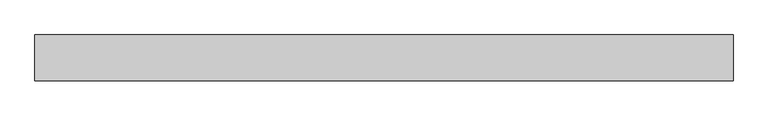
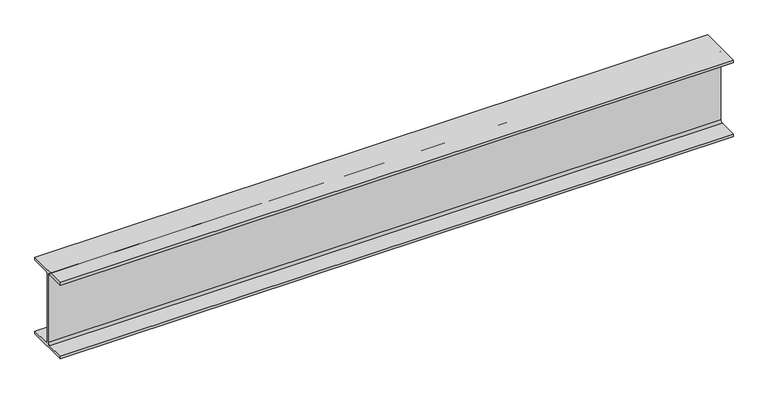
"""IFC4 building model written with IfcOpenShell, lengths in millimetres: beam geometry, Old_Steel Beam_H-KSD3502 : H_SB_ASB_H-482×300x11x15."""

from ifc_helpers import new_model, si_unit, point, frame, frame_2d, origin, place, context, project, spatial, polyline, circle_curve, trimmed, segment, composite_curve, outline, extrude, source, transform, mapped, element, save


def beam_420e2c5c(model_context):
    return source(origin(), model_context, "Body", "SweptSolid", [
        extrude(outline(composite_curve([segment(polyline([(82.5, -141.5), (82.5, -151.7), (-82.5, -151.7), (-82.5, -141.5), (-11.9, -141.5)]), True, "CONTINUOUS"), segment(trimmed(circle_curve(frame_2d((-11.9, -132.6)), 8.9), [point((-11.9, -141.5))], [point((-3.0, -132.6))], True, "CARTESIAN"), True, "CONTINUOUS"), segment(polyline([(-3.0, -132.6), (-3.0, 132.6)]), True, "CONTINUOUS"), segment(trimmed(circle_curve(frame_2d((-11.9, 132.6)), 8.9), [point((-3.0, 132.6))], [point((-11.9, 141.5))], True, "CARTESIAN"), True, "CONTINUOUS"), segment(polyline([(-11.9, 141.5), (-82.5, 141.5), (-82.5, 151.7), (82.5, 151.7), (82.5, 141.5), (11.9, 141.5)]), True, "CONTINUOUS"), segment(trimmed(circle_curve(frame_2d((11.9, 132.6)), 8.9), [point((11.9, 141.5))], [point((3.0, 132.6))], True, "CARTESIAN"), True, "CONTINUOUS"), segment(polyline([(3.0, 132.6), (3.0, -132.6)]), True, "CONTINUOUS"), segment(trimmed(circle_curve(frame_2d((11.9, -132.6)), 8.9), [point((3.0, -132.6))], [point((11.9, -141.5))], True, "CARTESIAN"), True, "CONTINUOUS"), segment(polyline([(11.9, -141.5), (82.5, -141.5)]), True, "CONTINUOUS")], self_intersect=False)), frame((-1254.8, 0.0, 0.0), z_axis=(1.0, 0.0, 0.0), x_axis=(0.0, 1.0, 0.0)), (0.0, 0.0, 1.0), 2522.3),
    ])


if __name__ == "__main__":
    model = new_model("IFC4")
    model_context = context("Model", 3, world=origin())
    ifc_project = project(units=[si_unit("LENGTHUNIT", "METRE", prefix="MILLI")], contexts=[model_context])
    site = spatial("IfcSite", under=ifc_project)
    building = spatial("IfcBuilding", under=site)
    placement = place(None, origin())
    beam_shape = beam_420e2c5c(model_context)
    element("IfcBeam", 1, ObjectType="Old_Steel Beam_H-KSD3502 : H_SB_ASB_H-482×300x11x15", at=placement, inside=building, context=model_context, shape_type="MappedRepresentation", body=[
        mapped(beam_shape, transform((0.0, 0.0, 0.0), x_axis=(1.0, 0.0, 0.0), y_axis=(0.0, 1.0, 0.0), z_axis=(0.0, 0.0, 1.0))),
    ])
    save(model, "model.ifc")

# Revit data of these elements
# Type "Old_Steel Beam_H-KSD3502 : H_SB_ASB_H-482×300x11x15"
#   Width = 30.0 cm
#   Web Thickness = 1.1 cm
#   Web Fillet = 2.6 cm
#   Warping Constant = 3680250.0 cm⁶
#   Torsional Moment of Inertia = 88.2192 cm⁴
#   Torsional Modulus = 1.0 cm³
#   Section Area = 145.5 cm²
#   Plastic Modulus weak axis = 695.0 cm³
#   Plastic Modulus strong axis = 2790.0 cm³
#   Perimeter = 2.10 m²/m
#   Nominal Weight = 114.00 kgf/m
#   Moment of Inertia weak axis = 6760.00 cm⁴
#   Moment of Inertia strong axis = 60400.00 cm⁴
#   Height = 48.2 cm
#   Flange Thickness = 1.5 cm
#   Elastic Modulus weak axis = 451.0 cm³
#   Elastic Modulus strong axis = 2500.0 cm³
#   Centroid Vertical = 24.1 cm
#   Centroid Horizontal = 15.0 cm
#   Length [instance default] = 1.5240 m
#   Structural Material [instance default] = Steel, 45-345
#   Assembly Code = ""
# Element 1 (IfcBeam, "Old_Steel Beam_H-KSD3502 : H_SB_ASB_H-482×300x11x15")
#   Structural Material = none
# Materials
#   "Steel, 45-345": class "Metal", colour RGB 189 187 185, transparency 0, Description = "Steel 345 MPa", Cost = 0
